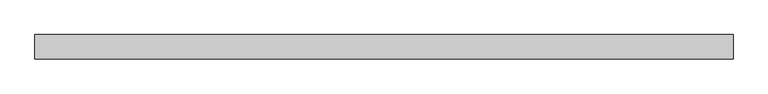
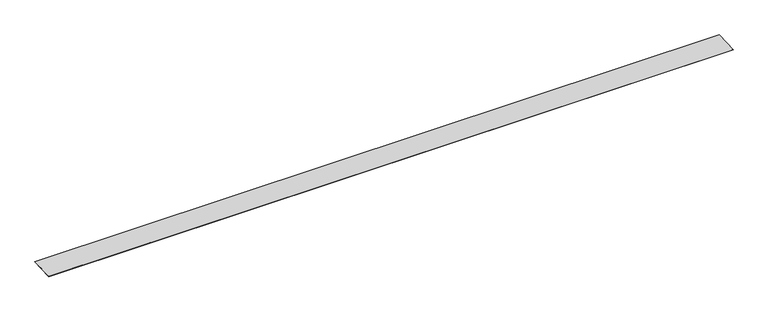
"""IFC4 building model written with IfcOpenShell, lengths in millimetres: proxy geometry, Generic Models 7:Generic Models 1:8:Generic Models 1:8 : Generic Models 7:Generic Models 1:337419:21 : Generic Models 7:Generic Models 1:8:Generic Models 1:8 : Generic Models 7:Generic Models 1:337419:315935."""

from ifc_helpers import new_model, si_unit, frame, origin, place, context, project, spatial, polyline, outline, extrude, source, transform, mapped, element, save


def generic_models_d3ff8a95(model_context):
    return source(origin(), model_context, "Body", "SweptSolid", [
        extrude(outline(polyline([(0.0, -171.0275031), (0.0, 0.0), (4876.8, 0.0), (4876.8, -171.0275031), (0.0, -171.0275031)])), frame((596182.8367242, -536663.130594, 10091.7535317), z_axis=(0.0, -0.04163054470947192, 0.9991330730924649), x_axis=(-1.0, 0.0, 0.0)), (0.0, 0.0, 1.0), 2.778125),
    ])


if __name__ == "__main__":
    model = new_model("IFC4")
    model_context = context("Model", 3, world=origin())
    ifc_project = project(units=[si_unit("LENGTHUNIT", "METRE", prefix="MILLI")], contexts=[model_context])
    site = spatial("IfcSite", under=ifc_project)
    building = spatial("IfcBuilding", under=site)
    placement = place(None, origin())
    generic_models_shape = generic_models_d3ff8a95(model_context)
    element("IfcBuildingElementProxy", 1, Name="Generic Models 7:Generic Models 1:8:Generic Models 1:8 : Generic Models 7:Generic Models 1:337419:21 : Generic Models 7:Generic Models 1:8:Generic Models 1:8 : Generic Models 7:Generic Models 1:337419:315935", ObjectType="Generic Models 7:Generic Models 1:8:Generic Models 1:8 : Generic Models 7:Generic Models 1:337419:21 : Generic Models 7:Generic Models 1:8:Generic Models 1:8 : Generic Models 7:Generic Models 1:337419:315935", at=placement, inside=building, context=model_context, shape_type="MappedRepresentation", body=[
        mapped(generic_models_shape, transform((0.0, 0.0, 0.0), x_axis=(1.0, 0.0, 0.0), y_axis=(0.0, 1.0, 0.0), z_axis=(0.0, 0.0, 1.0))),
    ])
    save(model, "model.ifc")

# Revit data of these elements
# Type "Generic Models 7:Generic Models 1:8:Generic Models 1:8 : Generic Models 7:Generic Models 1:337419:21 : Generic Models 7:Generic Models 1:8:Generic Models 1:8 : Generic Models 7:Generic Models 1:337419:315935"
#   NameOverride = "Generic Models 7:Generic Models 1:8:Generic Models 1:8 : Generic Models 7:Generic Models 1:337419:315935"
#   ObjectTypeOverride = "Generic Models 1:8 : Generic Models 7:Generic Models 1:337419"
#   Reference = "Generic Models 1"
#   Tag = "315935"
# Element 1 (IfcBuildingElementProxy, "Generic Models 7:Generic Models 1:8:Generic Models 1:8 : Generic Models 7:Generic Models 1:337419:21 : Generic Models 7:Generic Models 1:8:Generic Models 1:8 : Generic Models 7:Generic Models 1:337419:315935")
#   Materials on its faces: "STEEL PLATE FOR STOREFRONT SUPPORT T.B.D."
# Materials
#   "STEEL PLATE FOR STOREFRONT SUPPORT T.B.D.": class "Metal", colour RGB 189 187 185, transparency 0, Description = "Structural steel 50ksi", Cost = 0
